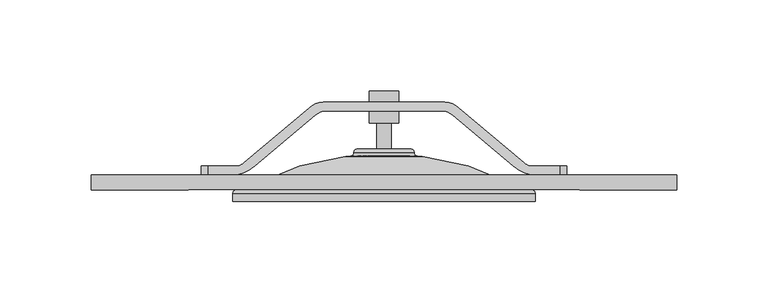
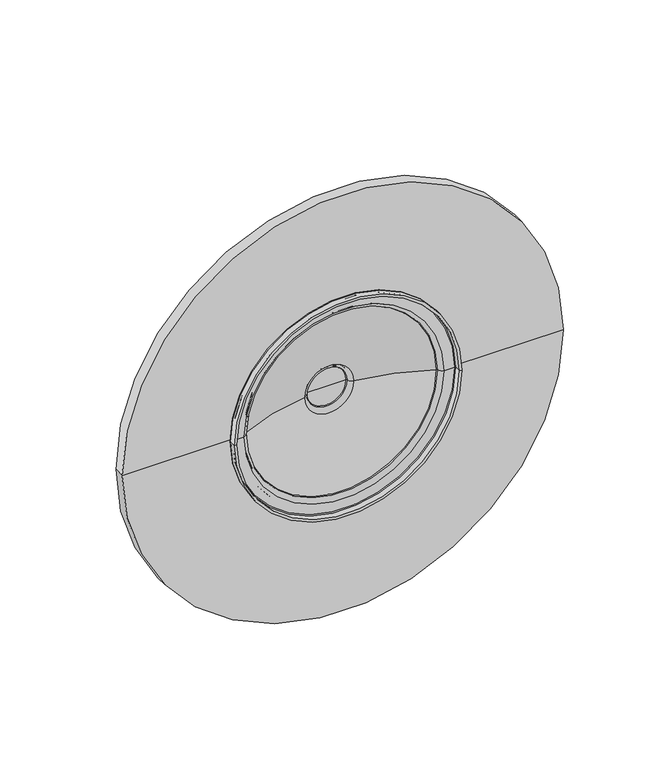
"""IFC4 building model written with IfcOpenShell, lengths in millimetres: proxy geometry, BVNC 300 8Y. : BVNC 300 8Y."""

from ifc_helpers import new_model, si_unit, point, frame, origin, place, context, project, spatial, polyline, circle_curve, ellipse_curve, trimmed, source, transform, mapped, element, save
from ifc_brep_helpers import plane_surface, cylinder_surface, revolved_surface, advanced_brep


def mechanical_equipment_0f1aea58(model_context):
    return source(origin(), model_context, "Body", "AdvancedBrep", [
        advanced_brep(
        [(44.3795006, 108.0, 2710.0), (54.2298211, 113.0, 2710.0), (87.44309, 140.8692417, 2710.0), (91.8102497, 143.0, 2710.0), (125.0, 143.0, 2710.0), (158.1897503, 143.0, 2710.0), (162.55691, 140.8692417, 2710.0), (195.7701789, 113.0, 2710.0), (205.6204994, 108.0, 2710.0), (221.2200072, 108.0, 2710.0), (221.2200072, 113.0, 2710.0), (205.6204994, 113.0, 2710.0), (201.5540671, 114.8851429, 2710.0), (165.874925, 144.8234979, 2710.0), (158.1897503, 148.0, 2710.0), (125.0, 148.0, 2710.0), (91.8102497, 148.0, 2710.0), (84.125075, 144.8234979, 2710.0), (48.4459329, 114.8851429, 2710.0), (44.3795006, 113.0, 2710.0), (28.7799928, 113.0, 2710.0), (28.7799928, 108.0, 2710.0), (44.3795006, 113.0, 2690.0), (48.4459329, 114.8851429, 2690.0), (84.125075, 144.8234979, 2690.0), (91.8102497, 148.0, 2690.0), (125.0, 148.0, 2690.0), (158.1897503, 148.0, 2690.0), (165.874925, 144.8234979, 2690.0), (201.5540671, 114.8851429, 2690.0), (205.6204994, 113.0, 2690.0), (221.2200072, 113.0, 2690.0), (221.2200072, 108.0, 2690.0), (205.6204994, 108.0, 2690.0), (195.7701789, 113.0, 2690.0), (162.55691, 140.8692417, 2690.0), (158.1897503, 143.0, 2690.0), (125.0, 143.0, 2690.0), (91.8102497, 143.0, 2690.0), (87.44309, 140.8692417, 2690.0), (54.2298211, 113.0, 2690.0), (44.3795006, 108.0, 2690.0), (28.7799928, 108.0, 2690.0), (28.7799928, 113.0, 2690.0), (25.0, 108.0, 2706.2200072), (25.0, 108.0, 2693.7799928), (225.0, 108.0, 2693.7799928), (225.0, 108.0, 2706.2200072), (225.0, 113.0, 2693.7799928), (225.0, 113.0, 2706.2200072), (25.0, 113.0, 2693.7799928), (25.0, 113.0, 2706.2200072)],
        [
            (0, 1, circle_curve(frame((38.5511411, 131.6851233, 2710.0), z_axis=(0.0, 0.0, 1.0), x_axis=(1.0, 0.0, 0.0)), 24.3916961)),
            (1, 2),
            (2, 3, circle_curve(frame((93.9022065, 133.1715663, 2710.0), z_axis=(0.0, 0.0, -1.0), x_axis=(1.0, 0.0, 0.0)), 10.0486015)),
            (3, 4),
            (4, 5),
            (5, 6, circle_curve(frame((156.0977935, 133.1715663, 2710.0), z_axis=(0.0, 0.0, -1.0), x_axis=(-1.0, 0.0, 0.0)), 10.0486015)),
            (6, 7),
            (7, 8, circle_curve(frame((211.4488589, 131.6851233, 2710.0), z_axis=(0.0, 0.0, 1.0), x_axis=(-1.0, 0.0, 0.0)), 24.3916961)),
            (8, 9),
            (9, 10),
            (10, 11),
            (11, 12, circle_curve(frame((205.6204994, 118.3284116, 2710.0), z_axis=(0.0, 0.0, -1.0), x_axis=(-1.0, 0.0, 0.0)), 5.3284116)),
            (12, 13),
            (13, 14, circle_curve(frame((158.1897503, 137.115059, 2710.0), z_axis=(0.0, 0.0, 1.0), x_axis=(-1.0, 0.0, 0.0)), 10.884941)),
            (14, 15),
            (15, 16),
            (16, 17, circle_curve(frame((91.8102497, 137.115059, 2710.0), z_axis=(0.0, 0.0, 1.0), x_axis=(1.0, 0.0, 0.0)), 10.884941)),
            (17, 18),
            (18, 19, circle_curve(frame((44.3795006, 118.3284116, 2710.0), z_axis=(0.0, 0.0, -1.0), x_axis=(1.0, 0.0, 0.0)), 5.3284116)),
            (19, 20),
            (20, 21),
            (21, 0),
            (22, 23, circle_curve(frame((44.3795006, 118.3284116, 2690.0), z_axis=(0.0, 0.0, 1.0), x_axis=(1.0, 0.0, 0.0)), 5.3284116)),
            (23, 24),
            (24, 25, circle_curve(frame((91.8102497, 137.115059, 2690.0), z_axis=(0.0, 0.0, -1.0), x_axis=(1.0, 0.0, 0.0)), 10.884941)),
            (25, 26),
            (26, 27),
            (27, 28, circle_curve(frame((158.1897503, 137.115059, 2690.0), z_axis=(0.0, 0.0, -1.0), x_axis=(-1.0, 0.0, 0.0)), 10.884941)),
            (28, 29),
            (29, 30, circle_curve(frame((205.6204994, 118.3284116, 2690.0), z_axis=(0.0, 0.0, 1.0), x_axis=(-1.0, 0.0, 0.0)), 5.3284116)),
            (30, 31),
            (31, 32),
            (32, 33),
            (33, 34, circle_curve(frame((211.4488589, 131.6851233, 2690.0), z_axis=(0.0, 0.0, -1.0), x_axis=(-1.0, 0.0, 0.0)), 24.3916961)),
            (34, 35),
            (35, 36, circle_curve(frame((156.0977935, 133.1715663, 2690.0), z_axis=(0.0, 0.0, 1.0), x_axis=(-1.0, 0.0, 0.0)), 10.0486015)),
            (36, 37),
            (37, 38),
            (38, 39, circle_curve(frame((93.9022065, 133.1715663, 2690.0), z_axis=(0.0, 0.0, 1.0), x_axis=(1.0, 0.0, 0.0)), 10.0486015)),
            (39, 40),
            (40, 41, circle_curve(frame((38.5511411, 131.6851233, 2690.0), z_axis=(0.0, 0.0, -1.0), x_axis=(1.0, 0.0, 0.0)), 24.3916961)),
            (41, 42),
            (42, 43),
            (43, 22),
            (41, 0),
            (21, 44, circle_curve(frame((28.7799928, 108.0, 2706.2200072), z_axis=(0.0, -1.0, 0.0), x_axis=(1.0, 0.0, 0.0)), 3.7799928)),
            (44, 45),
            (45, 42, circle_curve(frame((28.7799928, 108.0, 2693.7799928), z_axis=(0.0, -1.0, 0.0), x_axis=(1.0, 0.0, 0.0)), 3.7799928)),
            (40, 1),
            (39, 2),
            (38, 3),
            (37, 4),
            (36, 5),
            (35, 6),
            (34, 7),
            (33, 8),
            (32, 46, circle_curve(frame((221.2200072, 108.0, 2693.7799928), z_axis=(0.0, -1.0, 0.0), x_axis=(-1.0, 0.0, 0.0)), 3.7799928)),
            (46, 47),
            (47, 9, circle_curve(frame((221.2200072, 108.0, 2706.2200072), z_axis=(0.0, -1.0, 0.0), x_axis=(-1.0, 0.0, 0.0)), 3.7799928)),
            (46, 48),
            (48, 49),
            (49, 47),
            (30, 11),
            (10, 49, circle_curve(frame((221.2200072, 113.0, 2706.2200072), z_axis=(0.0, 1.0, 0.0), x_axis=(-1.0, 0.0, 0.0)), 3.7799928)),
            (48, 31, circle_curve(frame((221.2200072, 113.0, 2693.7799928), z_axis=(0.0, 1.0, 0.0), x_axis=(-1.0, 0.0, 0.0)), 3.7799928)),
            (29, 12),
            (28, 13),
            (27, 14),
            (26, 15),
            (25, 16),
            (24, 17),
            (23, 18),
            (22, 19),
            (43, 50, circle_curve(frame((28.7799928, 113.0, 2693.7799928), z_axis=(0.0, 1.0, 0.0), x_axis=(1.0, 0.0, 0.0)), 3.7799928)),
            (50, 51),
            (51, 20, circle_curve(frame((28.7799928, 113.0, 2706.2200072), z_axis=(0.0, 1.0, 0.0), x_axis=(1.0, 0.0, 0.0)), 3.7799928)),
            (44, 51),
            (50, 45),
        ],
        [
            plane_surface(frame((25.0, 108.0, 2710.0), z_axis=(0.0, 0.0, 1.0), x_axis=(1.0, 0.0, 0.0))),
            plane_surface(frame((25.0, 108.0, 2690.0), z_axis=(0.0, 0.0, -1.0), x_axis=(-1.0, 0.0, 0.0))),
            plane_surface(frame((25.0, 108.0, 2710.0), z_axis=(0.0, -1.0, 0.0), x_axis=(0.0, 0.0, -1.0))),
            cylinder_surface(frame((38.5511411, 131.6851233, 2690.0), z_axis=(0.0, 0.0, 1.0), x_axis=(1.0, 0.0, 0.0)), 24.3916961),
            plane_surface(frame((54.2298211, 113.0, 2710.0), z_axis=(0.6427876096865391, -0.7660444431189783, 0.0), x_axis=(0.0, 0.0, -1.0))),
            revolved_surface(polyline([(103.95080800000001, 133.1715663, 2690.0), (103.95080800000001, 133.1715663, 2710.0)]), (93.9022065, 133.1715663, 2690.0), (0.0, 0.0, -1.0)),
            plane_surface(frame((91.8102497, 143.0, 2710.0), z_axis=(0.0, -1.0, 0.0), x_axis=(0.0, 0.0, -1.0))),
            plane_surface(frame((125.0, 143.0, 2710.0), z_axis=(0.0, -1.0, 0.0), x_axis=(0.0, 0.0, -1.0))),
            revolved_surface(polyline([(146.049192, 133.1715663, 2690.0), (146.049192, 133.1715663, 2710.0)]), (156.0977935, 133.1715663, 2690.0), (0.0, 0.0, -1.0)),
            plane_surface(frame((162.55691, 140.8692417, 2710.0), z_axis=(-0.6427876096865387, -0.7660444431189786, 0.0), x_axis=(0.0, 0.0, -1.0))),
            cylinder_surface(frame((211.4488589, 131.6851233, 2690.0), z_axis=(0.0, 0.0, 1.0), x_axis=(-1.0, 0.0, 0.0)), 24.3916961),
            plane_surface(frame((205.6204994, 108.0, 2710.0), z_axis=(0.0, -1.0, 0.0), x_axis=(0.0, 0.0, -1.0))),
            plane_surface(frame((225.0, 108.0, 2710.0), z_axis=(1.0, 0.0, 0.0), x_axis=(0.0, 0.0, -1.0))),
            plane_surface(frame((225.0, 113.0, 2710.0), z_axis=(0.0, 1.0, 0.0), x_axis=(0.0, 0.0, -1.0))),
            revolved_surface(polyline([(200.2920878, 118.3284116, 2690.0), (200.2920878, 118.3284116, 2710.0)]), (205.6204994, 118.3284116, 2690.0), (0.0, 0.0, -1.0)),
            plane_surface(frame((201.5540671, 114.8851429, 2710.0), z_axis=(0.6427876096865414, 0.7660444431189763, 0.0), x_axis=(0.0, 0.0, -1.0))),
            cylinder_surface(frame((158.1897503, 137.115059, 2690.0), z_axis=(0.0, 0.0, 1.0), x_axis=(-1.0, 0.0, 0.0)), 10.884941),
            plane_surface(frame((158.1897503, 148.0, 2710.0), z_axis=(0.0, 1.0, 0.0), x_axis=(0.0, 0.0, -1.0))),
            plane_surface(frame((125.0, 148.0, 2710.0), z_axis=(0.0, 1.0, 0.0), x_axis=(0.0, 0.0, -1.0))),
            cylinder_surface(frame((91.8102497, 137.115059, 2690.0), z_axis=(0.0, 0.0, 1.0), x_axis=(1.0, 0.0, 0.0)), 10.884941),
            plane_surface(frame((84.125075, 144.8234979, 2710.0), z_axis=(-0.6427876096865359, 0.766044443118981, 0.0), x_axis=(0.0, 0.0, -1.0))),
            revolved_surface(polyline([(49.7079122, 118.3284116, 2690.0), (49.7079122, 118.3284116, 2710.0)]), (44.3795006, 118.3284116, 2690.0), (0.0, 0.0, -1.0)),
            plane_surface(frame((44.3795006, 113.0, 2710.0), z_axis=(0.0, 1.0, 0.0), x_axis=(0.0, 0.0, -1.0))),
            plane_surface(frame((25.0, 113.0, 2710.0), z_axis=(-1.0, 0.0, 0.0), x_axis=(0.0, 0.0, -1.0))),
            cylinder_surface(frame((28.7799928, 108.0, 2693.7799928), z_axis=(0.0, -1.0, 0.0), x_axis=(1.0, 0.0, 0.0)), 3.7799928),
            cylinder_surface(frame((28.7799928, 93.5, 2706.2200072), z_axis=(0.0, -1.0, 0.0), x_axis=(1.0, 0.0, 0.0)), 3.7799928),
            cylinder_surface(frame((221.2200072, 93.5, 2693.7799928), z_axis=(0.0, -1.0, 0.0), x_axis=(-1.0, 0.0, 0.0)), 3.7799928),
            cylinder_surface(frame((221.2200072, 93.5, 2706.2200072), z_axis=(0.0, -1.0, 0.0), x_axis=(-1.0, 0.0, 0.0)), 3.7799928),
        ],
        [
            (0, [[1, 2, 3, 4, 5, 6, 7, 8, 9, 10, 11, 12, 13, 14, 15, 16, 17, 18, 19, 20, 21, 22]]),
            (1, [[23, 24, 25, 26, 27, 28, 29, 30, 31, 32, 33, 34, 35, 36, 37, 38, 39, 40, 41, 42, 43, 44]]),
            (2, [[45, -22, 46, 47, 48, -42]]),
            (3, [[-1, -45, -41, 49]]),
            (4, [[-2, -49, -40, 50]]),
            (5, [[-3, -50, -39, 51]]),
            (6, [[-4, -51, -38, 52]]),
            (7, [[-5, -52, -37, 53]]),
            (8, [[-6, -53, -36, 54]]),
            (9, [[-7, -54, -35, 55]]),
            (10, [[-8, -55, -34, 56]]),
            (11, [[-56, -33, 57, 58, 59, -9]]),
            (12, [[-58, 60, 61, 62]]),
            (13, [[63, -11, 64, -61, 65, -31]]),
            (14, [[-12, -63, -30, 66]]),
            (15, [[-13, -66, -29, 67]]),
            (16, [[-14, -67, -28, 68]]),
            (17, [[-15, -68, -27, 69]]),
            (18, [[-16, -69, -26, 70]]),
            (19, [[-17, -70, -25, 71]]),
            (20, [[-18, -71, -24, 72]]),
            (21, [[-19, -72, -23, 73]]),
            (22, [[-73, -44, 74, 75, 76, -20]]),
            (23, [[-47, 77, -75, 78]]),
            (24, [[-43, -48, -78, -74]]),
            (25, [[-21, -76, -77, -46]]),
            (26, [[-32, -65, -60, -57]]),
            (27, [[-10, -59, -62, -64]]),
        ],
    ),
        advanced_brep(
        [(207.7271571, 93.5, 2700.0), (42.2728429, 93.5, 2700.0), (42.2728429, 97.7728429, 2700.0), (207.7271571, 97.7728429, 2700.0), (205.9367462, 93.5, 2700.0), (44.0632538, 93.5, 2700.0), (205.9367462, 97.9071057, 2700.0), (44.0632538, 97.9071057, 2700.0), (205.3438519, 98.5, 2700.0), (44.6561481, 98.5, 2700.0), (197.7785514, 98.5, 2700.0), (52.2214486, 98.5, 2700.0), (194.5390342, 101.1233093, 2700.0), (55.4609658, 101.1233093, 2700.0), (194.110594, 101.9290881, 2700.0), (55.889406, 101.9290881, 2700.0), (143.1174907, 117.056758, 2700.0), (106.8825093, 117.056758, 2700.0), (139.9690463, 120.2052024, 2700.0), (110.0309537, 120.2052024, 2700.0), (139.3942487, 120.78, 2700.0), (110.6057513, 120.78, 2700.0), (125.0, 120.78, 2700.0), (139.6388233, 122.2731901, 2700.0), (110.3611767, 122.2731901, 2700.0), (120.9566338, 122.2731901, 2700.0), (129.0433662, 122.2731901, 2700.0), (141.5029828, 120.4090307, 2700.0), (108.4970172, 120.4090307, 2700.0), (143.1991524, 118.522856, 2700.0), (106.8008476, 118.522856, 2700.0), (145.9642188, 118.2410596, 2700.0), (104.0357812, 118.2410596, 2700.0), (194.877574, 103.206216, 2700.0), (55.122426, 103.206216, 2700.0), (196.1038029, 101.6367146, 2700.0), (53.8961971, 101.6367146, 2700.0), (198.0543634, 100.0, 2700.0), (51.9456366, 100.0, 2700.0), (200.0, 100.0, 2700.0), (50.0, 100.0, 2700.0), (200.0, 108.0, 2700.0), (50.0, 108.0, 2700.0), (285.0, 108.0, 2700.0), (-35.0, 108.0, 2700.0), (285.0, 100.0, 2700.0), (-35.0, 100.0, 2700.0), (205.5, 100.0, 2700.0), (44.5, 100.0, 2700.0), (133.0867323, 136.6576943, 2700.0), (116.9132677, 136.6576943, 2700.0), (116.9132677, 153.9, 2700.0), (133.0867323, 153.9, 2700.0), (129.0433662, 136.6576943, 2700.0), (120.9566338, 136.6576943, 2700.0), (125.0, 153.9, 2700.0)],
        [
            (0, 1, circle_curve(frame((125.0, 93.5, 2700.0), z_axis=(0.0, 1.0, 0.0), x_axis=(-1.0, 0.0, 0.0)), 82.7271571)),
            (1, 2),
            (2, 3, circle_curve(frame((125.0, 97.7728429, 2700.0), z_axis=(0.0, -1.0, 0.0), x_axis=(-1.0, 0.0, 0.0)), 82.7271571)),
            (3, 0),
            (1, 0, circle_curve(frame((125.0, 93.5, 2700.0), z_axis=(0.0, 1.0, 0.0), x_axis=(-1.0, 0.0, 0.0)), 82.7271571)),
            (3, 2, circle_curve(frame((125.0, 97.7728429, 2700.0), z_axis=(0.0, -1.0, 0.0), x_axis=(-1.0, 0.0, 0.0)), 82.7271571)),
            (0, 4),
            (4, 5, circle_curve(frame((125.0, 93.5, 2700.0), z_axis=(0.0, 1.0, 0.0), x_axis=(-1.0, 0.0, 0.0)), 80.9367462)),
            (5, 1),
            (5, 4, circle_curve(frame((125.0, 93.5, 2700.0), z_axis=(0.0, 1.0, 0.0), x_axis=(-1.0, 0.0, 0.0)), 80.9367462)),
            (4, 6),
            (6, 7, circle_curve(frame((125.0, 97.9071057, 2700.0), z_axis=(0.0, 1.0, 0.0), x_axis=(-1.0, 0.0, 0.0)), 80.9367462)),
            (7, 5),
            (7, 6, circle_curve(frame((125.0, 97.9071057, 2700.0), z_axis=(0.0, 1.0, 0.0), x_axis=(-1.0, 0.0, 0.0)), 80.9367462)),
            (6, 8, circle_curve(frame((205.3438519, 97.9071057, 2700.0), z_axis=(0.0, 0.0, 1.0), x_axis=(-1.0, 0.0, 0.0)), 0.5928943)),
            (8, 9, circle_curve(frame((125.0, 98.5, 2700.0), z_axis=(0.0, 1.0, 0.0), x_axis=(-1.0, 0.0, 0.0)), 80.3438519)),
            (9, 7, circle_curve(frame((44.6561481, 97.9071057, 2700.0), z_axis=(0.0, 0.0, 1.0), x_axis=(1.0, 0.0, 0.0)), 0.5928943)),
            (9, 8, circle_curve(frame((125.0, 98.5, 2700.0), z_axis=(0.0, 1.0, 0.0), x_axis=(-1.0, 0.0, 0.0)), 80.3438519)),
            (8, 10),
            (10, 11, circle_curve(frame((125.0, 98.5, 2700.0), z_axis=(0.0, 1.0, 0.0), x_axis=(-1.0, 0.0, 0.0)), 72.7785514)),
            (11, 9),
            (11, 10, circle_curve(frame((125.0, 98.5, 2700.0), z_axis=(0.0, 1.0, 0.0), x_axis=(-1.0, 0.0, 0.0)), 72.7785514)),
            (10, 12, circle_curve(frame((197.9467336, 102.0195777, 2700.0), z_axis=(0.0, 0.0, -1.0), x_axis=(-1.0, 0.0, 0.0)), 3.5235937)),
            (12, 13, circle_curve(frame((125.0, 101.1233093, 2700.0), z_axis=(0.0, 1.0, 0.0), x_axis=(-1.0, 0.0, 0.0)), 69.5390342)),
            (13, 11, circle_curve(frame((52.0532664, 102.0195777, 2700.0), z_axis=(0.0, 0.0, -1.0), x_axis=(1.0, 0.0, 0.0)), 3.5235937)),
            (13, 12, circle_curve(frame((125.0, 101.1233093, 2700.0), z_axis=(0.0, 1.0, 0.0), x_axis=(-1.0, 0.0, 0.0)), 69.5390342)),
            (12, 14, circle_curve(frame((193.7458269, 101.2183458, 2700.0), z_axis=(0.0, 0.0, 1.0), x_axis=(-1.0, 0.0, 0.0)), 0.7988803)),
            (14, 15, circle_curve(frame((125.0, 101.9290881, 2700.0), z_axis=(0.0, 1.0, 0.0), x_axis=(-1.0, 0.0, 0.0)), 69.110594)),
            (15, 13, circle_curve(frame((56.2541731, 101.2183458, 2700.0), z_axis=(0.0, 0.0, 1.0), x_axis=(1.0, 0.0, 0.0)), 0.7988803)),
            (15, 14, circle_curve(frame((125.0, 101.9290881, 2700.0), z_axis=(0.0, 1.0, 0.0), x_axis=(-1.0, 0.0, 0.0)), 69.110594)),
            (14, 16, circle_curve(frame((128.3688639, -26.1675298, 2700.0), z_axis=(0.0, 0.0, 1.0), x_axis=(-1.0, 0.0, 0.0)), 143.9816606)),
            (16, 17, circle_curve(frame((125.0, 117.056758, 2700.0), z_axis=(0.0, 1.0, 0.0), x_axis=(-1.0, 0.0, 0.0)), 18.1174907)),
            (17, 15, circle_curve(frame((121.6311361, -26.1675298, 2700.0), z_axis=(0.0, 0.0, 1.0), x_axis=(1.0, 0.0, 0.0)), 143.9816606)),
            (17, 16, circle_curve(frame((125.0, 117.056758, 2700.0), z_axis=(0.0, 1.0, 0.0), x_axis=(-1.0, 0.0, 0.0)), 18.1174907)),
            (16, 18, circle_curve(frame((143.1174907, 120.2052024, 2700.0), z_axis=(0.0, 0.0, -1.0), x_axis=(-1.0, 0.0, 0.0)), 3.1484444)),
            (18, 19, circle_curve(frame((125.0, 120.2052024, 2700.0), z_axis=(0.0, 1.0, 0.0), x_axis=(-1.0, 0.0, 0.0)), 14.9690463)),
            (19, 17, circle_curve(frame((106.8825093, 120.2052024, 2700.0), z_axis=(0.0, 0.0, -1.0), x_axis=(1.0, 0.0, 0.0)), 3.1484444)),
            (19, 18, circle_curve(frame((125.0, 120.2052024, 2700.0), z_axis=(0.0, 1.0, 0.0), x_axis=(-1.0, 0.0, 0.0)), 14.9690463)),
            (18, 20, circle_curve(frame((139.3942487, 120.2052024, 2700.0), z_axis=(0.0, 0.0, 1.0), x_axis=(-1.0, 0.0, 0.0)), 0.5747976)),
            (20, 21, circle_curve(frame((125.0, 120.78, 2700.0), z_axis=(0.0, 1.0, 0.0), x_axis=(-1.0, 0.0, 0.0)), 14.3942487)),
            (21, 19, circle_curve(frame((110.6057513, 120.2052024, 2700.0), z_axis=(0.0, 0.0, 1.0), x_axis=(1.0, 0.0, 0.0)), 0.5747976)),
            (21, 20, circle_curve(frame((125.0, 120.78, 2700.0), z_axis=(0.0, 1.0, 0.0), x_axis=(-1.0, 0.0, 0.0)), 14.3942487)),
            (20, 22),
            (22, 21),
            (23, 24, circle_curve(frame((125.0, 122.2731901, 2700.0), z_axis=(0.0, 1.0, 0.0), x_axis=(-1.0, 0.0, 0.0)), 14.6388233)),
            (24, 25),
            (25, 26, circle_curve(frame((125.0, 122.2731901, 2700.0), z_axis=(0.0, -1.0, 0.0), x_axis=(-1.0, 0.0, 0.0)), 4.0433662)),
            (26, 23),
            (24, 23, circle_curve(frame((125.0, 122.2731901, 2700.0), z_axis=(0.0, 1.0, 0.0), x_axis=(-1.0, 0.0, 0.0)), 14.6388233)),
            (26, 25, circle_curve(frame((125.0, 122.2731901, 2700.0), z_axis=(0.0, -1.0, 0.0), x_axis=(-1.0, 0.0, 0.0)), 4.0433662)),
            (23, 27, circle_curve(frame((139.6388233, 120.4090307, 2700.0), z_axis=(0.0, 0.0, -1.0), x_axis=(-1.0, 0.0, 0.0)), 1.8641595)),
            (27, 28, circle_curve(frame((125.0, 120.4090307, 2700.0), z_axis=(0.0, 1.0, 0.0), x_axis=(-1.0, 0.0, 0.0)), 16.5029828)),
            (28, 24, circle_curve(frame((110.3611767, 120.4090307, 2700.0), z_axis=(0.0, 0.0, -1.0), x_axis=(1.0, 0.0, 0.0)), 1.8641595)),
            (28, 27, circle_curve(frame((125.0, 120.4090307, 2700.0), z_axis=(0.0, 1.0, 0.0), x_axis=(-1.0, 0.0, 0.0)), 16.5029828)),
            (27, 29, circle_curve(frame((143.3997997, 120.4090307, 2700.0), z_axis=(0.0, 0.0, 1.0), x_axis=(-1.0, 0.0, 0.0)), 1.8968169)),
            (29, 30, circle_curve(frame((125.0, 118.522856, 2700.0), z_axis=(0.0, 1.0, 0.0), x_axis=(-1.0, 0.0, 0.0)), 18.1991524)),
            (30, 28, circle_curve(frame((106.6002003, 120.4090307, 2700.0), z_axis=(0.0, 0.0, 1.0), x_axis=(1.0, 0.0, 0.0)), 1.8968169)),
            (30, 29, circle_curve(frame((125.0, 118.522856, 2700.0), z_axis=(0.0, 1.0, 0.0), x_axis=(-1.0, 0.0, 0.0)), 18.1991524)),
            (29, 31, circle_curve(frame((176.4809645, 431.386753, 2700.0), z_axis=(0.0, 0.0, 1.0), x_axis=(-1.0, 0.0, 0.0)), 314.6291421)),
            (31, 32, circle_curve(frame((125.0, 118.2410596, 2700.0), z_axis=(0.0, 1.0, 0.0), x_axis=(-1.0, 0.0, 0.0)), 20.9642188)),
            (32, 30, circle_curve(frame((73.5190355, 431.386753, 2700.0), z_axis=(0.0, 0.0, 1.0), x_axis=(1.0, 0.0, 0.0)), 314.6291421)),
            (32, 31, circle_curve(frame((125.0, 118.2410596, 2700.0), z_axis=(0.0, 1.0, 0.0), x_axis=(-1.0, 0.0, 0.0)), 20.9642188)),
            (31, 33, circle_curve(frame((131.9555378, -14.4169888, 2700.0), z_axis=(0.0, 0.0, -1.0), x_axis=(-1.0, 0.0, 0.0)), 133.3956557)),
            (33, 34, circle_curve(frame((125.0, 103.206216, 2700.0), z_axis=(0.0, 1.0, 0.0), x_axis=(-1.0, 0.0, 0.0)), 69.877574)),
            (34, 32, circle_curve(frame((118.0444622, -14.4169888, 2700.0), z_axis=(0.0, 0.0, -1.0), x_axis=(1.0, 0.0, 0.0)), 133.3956557)),
            (34, 33, circle_curve(frame((125.0, 103.206216, 2700.0), z_axis=(0.0, 1.0, 0.0), x_axis=(-1.0, 0.0, 0.0)), 69.877574)),
            (33, 35, circle_curve(frame((194.0147871, 101.2683648, 2700.0), z_axis=(0.0, 0.0, -1.0), x_axis=(-1.0, 0.0, 0.0)), 2.1212422)),
            (35, 36, circle_curve(frame((125.0, 101.6367146, 2700.0), z_axis=(0.0, 1.0, 0.0), x_axis=(-1.0, 0.0, 0.0)), 71.1038029)),
            (36, 34, circle_curve(frame((55.9852129, 101.2683648, 2700.0), z_axis=(0.0, 0.0, -1.0), x_axis=(1.0, 0.0, 0.0)), 2.1212422)),
            (36, 35, circle_curve(frame((125.0, 101.6367146, 2700.0), z_axis=(0.0, 1.0, 0.0), x_axis=(-1.0, 0.0, 0.0)), 71.1038029)),
            (35, 37, circle_curve(frame((198.0543634, 101.9806511, 2700.0), z_axis=(0.0, 0.0, 1.0), x_axis=(-1.0, 0.0, 0.0)), 1.9806511)),
            (37, 38, circle_curve(frame((125.0, 100.0, 2700.0), z_axis=(0.0, 1.0, 0.0), x_axis=(-1.0, 0.0, 0.0)), 73.0543634)),
            (38, 36, circle_curve(frame((51.9456366, 101.9806511, 2700.0), z_axis=(0.0, 0.0, 1.0), x_axis=(1.0, 0.0, 0.0)), 1.9806511)),
            (38, 37, circle_curve(frame((125.0, 100.0, 2700.0), z_axis=(0.0, 1.0, 0.0), x_axis=(-1.0, 0.0, 0.0)), 73.0543634)),
            (37, 39),
            (39, 40, circle_curve(frame((125.0, 100.0, 2700.0), z_axis=(0.0, 1.0, 0.0), x_axis=(-1.0, 0.0, 0.0)), 75.0)),
            (40, 38),
            (40, 39, circle_curve(frame((125.0, 100.0, 2700.0), z_axis=(0.0, 1.0, 0.0), x_axis=(-1.0, 0.0, 0.0)), 75.0)),
            (39, 41),
            (41, 42, circle_curve(frame((125.0, 108.0, 2700.0), z_axis=(0.0, 1.0, 0.0), x_axis=(-1.0, 0.0, 0.0)), 75.0)),
            (42, 40),
            (42, 41, circle_curve(frame((125.0, 108.0, 2700.0), z_axis=(0.0, 1.0, 0.0), x_axis=(-1.0, 0.0, 0.0)), 75.0)),
            (41, 43),
            (43, 44, circle_curve(frame((125.0, 108.0, 2700.0), z_axis=(0.0, 1.0, 0.0), x_axis=(-1.0, 0.0, 0.0)), 160.0)),
            (44, 42),
            (44, 43, circle_curve(frame((125.0, 108.0, 2700.0), z_axis=(0.0, 1.0, 0.0), x_axis=(-1.0, 0.0, 0.0)), 160.0)),
            (43, 45),
            (45, 46, circle_curve(frame((125.0, 100.0, 2700.0), z_axis=(0.0, 1.0, 0.0), x_axis=(-1.0, 0.0, 0.0)), 160.0)),
            (46, 44),
            (46, 45, circle_curve(frame((125.0, 100.0, 2700.0), z_axis=(0.0, 1.0, 0.0), x_axis=(-1.0, 0.0, 0.0)), 160.0)),
            (45, 47),
            (47, 48, circle_curve(frame((125.0, 100.0, 2700.0), z_axis=(0.0, 1.0, 0.0), x_axis=(-1.0, 0.0, 0.0)), 80.5)),
            (48, 46),
            (48, 47, circle_curve(frame((125.0, 100.0, 2700.0), z_axis=(0.0, 1.0, 0.0), x_axis=(-1.0, 0.0, 0.0)), 80.5)),
            (2, 48, circle_curve(frame((44.5, 97.7728429, 2700.0), z_axis=(0.0, 0.0, -1.0), x_axis=(1.0, 0.0, 0.0)), 2.2271571)),
            (47, 3, circle_curve(frame((205.5, 97.7728429, 2700.0), z_axis=(0.0, 0.0, -1.0), x_axis=(-1.0, 0.0, 0.0)), 2.2271571)),
            (49, 50, circle_curve(frame((125.0, 136.6576943, 2700.0), z_axis=(0.0, 1.0, 0.0), x_axis=(-1.0, 0.0, 0.0)), 8.0867323)),
            (50, 51),
            (51, 52, circle_curve(frame((125.0, 153.9, 2700.0), z_axis=(0.0, -1.0, 0.0), x_axis=(-1.0, 0.0, 0.0)), 8.0867323)),
            (52, 49),
            (50, 49, circle_curve(frame((125.0, 136.6576943, 2700.0), z_axis=(0.0, 1.0, 0.0), x_axis=(-1.0, 0.0, 0.0)), 8.0867323)),
            (52, 51, circle_curve(frame((125.0, 153.9, 2700.0), z_axis=(0.0, -1.0, 0.0), x_axis=(-1.0, 0.0, 0.0)), 8.0867323)),
            (49, 53),
            (53, 54, circle_curve(frame((125.0, 136.6576943, 2700.0), z_axis=(0.0, 1.0, 0.0), x_axis=(-1.0, 0.0, 0.0)), 4.0433662)),
            (54, 50),
            (54, 53, circle_curve(frame((125.0, 136.6576943, 2700.0), z_axis=(0.0, 1.0, 0.0), x_axis=(-1.0, 0.0, 0.0)), 4.0433662)),
            (51, 55),
            (55, 52),
            (25, 54),
            (53, 26),
        ],
        [
            cylinder_surface(frame((125.0, 193.5, 2700.0), z_axis=(0.0, -1.0, 0.0), x_axis=(-1.0, 0.0, 0.0)), 82.7271571),
            plane_surface(frame((125.0, 93.5, 2700.0), z_axis=(0.0, -1.0, 0.0), x_axis=(-1.0, 0.0, 0.0))),
            revolved_surface(polyline([(44.0632538, 93.5, 2700.0), (44.0632538, 97.9071057, 2700.0)]), (125.0, 193.5, 2700.0), (0.0, -1.0, 0.0)),
            revolved_surface(trimmed(ellipse_curve(frame((44.6561481, 97.9071057, 2700.0), z_axis=(0.0, 0.0, -1.0), x_axis=(1.0, 0.0, 0.0)), 0.5928943, 0.5928943), [point((44.0632538, 97.9071057, 2700.0))], [point((44.6561481, 98.5, 2700.0))], True, "CARTESIAN"), (125.0, 193.5, 2700.0), (0.0, -1.0, 0.0)),
            plane_surface(frame((125.0, 98.5, 2700.0), z_axis=(0.0, -1.0, 0.0), x_axis=(-1.0, 0.0, 0.0))),
            revolved_surface(trimmed(ellipse_curve(frame((52.0532664, 102.0195777, 2700.0), z_axis=(0.0, 0.0, 1.0), x_axis=(1.0, 0.0, 0.0)), 3.5235937, 3.5235937), [point((52.2214486, 98.5, 2700.0))], [point((55.4609658, 101.1233093, 2700.0))], True, "CARTESIAN"), (125.0, 193.5, 2700.0), (0.0, -1.0, 0.0)),
            revolved_surface(trimmed(ellipse_curve(frame((56.2541731, 101.2183458, 2700.0), z_axis=(0.0, 0.0, -1.0), x_axis=(1.0, 0.0, 0.0)), 0.7988803, 0.7988803), [point((55.4609658, 101.1233093, 2700.0))], [point((55.889406, 101.9290881, 2700.0))], True, "CARTESIAN"), (125.0, 193.5, 2700.0), (0.0, -1.0, 0.0)),
            revolved_surface(trimmed(ellipse_curve(frame((121.6311361, -26.1675298, 2700.0), z_axis=(0.0, 0.0, -1.0), x_axis=(1.0, 0.0, 0.0)), 143.9816606, 143.9816606), [point((55.889406, 101.9290881, 2700.0))], [point((106.8825093, 117.056758, 2700.0))], True, "CARTESIAN"), (125.0, 193.5, 2700.0), (0.0, -1.0, 0.0)),
            revolved_surface(trimmed(ellipse_curve(frame((106.8825093, 120.2052024, 2700.0), z_axis=(0.0, 0.0, 1.0), x_axis=(1.0, 0.0, 0.0)), 3.1484444, 3.1484444), [point((106.8825093, 117.056758, 2700.0))], [point((110.0309537, 120.2052024, 2700.0))], True, "CARTESIAN"), (125.0, 193.5, 2700.0), (0.0, -1.0, 0.0)),
            revolved_surface(trimmed(ellipse_curve(frame((110.6057513, 120.2052024, 2700.0), z_axis=(0.0, 0.0, -1.0), x_axis=(1.0, 0.0, 0.0)), 0.5747976, 0.5747976), [point((110.0309537, 120.2052024, 2700.0))], [point((110.6057513, 120.78, 2700.0))], True, "CARTESIAN"), (125.0, 193.5, 2700.0), (0.0, -1.0, 0.0)),
            plane_surface(frame((125.0, 120.78, 2700.0), z_axis=(0.0, -1.0, 0.0), x_axis=(-1.0, 0.0, 0.0))),
            plane_surface(frame((125.0, 122.2731901, 2700.0), z_axis=(0.0, 1.0, 0.0), x_axis=(-1.0, 0.0, 0.0))),
            revolved_surface(trimmed(ellipse_curve(frame((110.3611767, 120.4090307, 2700.0), z_axis=(0.0, 0.0, 1.0), x_axis=(1.0, 0.0, 0.0)), 1.8641595, 1.8641595), [point((110.3611767, 122.2731901, 2700.0))], [point((108.4970172, 120.4090307, 2700.0))], True, "CARTESIAN"), (125.0, 193.5, 2700.0), (0.0, -1.0, 0.0)),
            revolved_surface(trimmed(ellipse_curve(frame((106.6002003, 120.4090307, 2700.0), z_axis=(0.0, 0.0, -1.0), x_axis=(1.0, 0.0, 0.0)), 1.8968169, 1.8968169), [point((108.4970172, 120.4090307, 2700.0))], [point((106.8008476, 118.522856, 2700.0))], True, "CARTESIAN"), (125.0, 193.5, 2700.0), (0.0, -1.0, 0.0)),
            revolved_surface(trimmed(ellipse_curve(frame((73.5190355, 431.386753, 2700.0), z_axis=(0.0, 0.0, -1.0), x_axis=(1.0, 0.0, 0.0)), 314.6291421, 314.6291421), [point((106.8008476, 118.522856, 2700.0))], [point((104.0357812, 118.2410596, 2700.0))], True, "CARTESIAN"), (125.0, 193.5, 2700.0), (0.0, -1.0, 0.0)),
            revolved_surface(trimmed(ellipse_curve(frame((118.0444622, -14.4169888, 2700.0), z_axis=(0.0, 0.0, 1.0), x_axis=(1.0, 0.0, 0.0)), 133.3956557, 133.3956557), [point((104.0357812, 118.2410596, 2700.0))], [point((55.122426, 103.206216, 2700.0))], True, "CARTESIAN"), (125.0, 193.5, 2700.0), (0.0, -1.0, 0.0)),
            revolved_surface(trimmed(ellipse_curve(frame((55.9852129, 101.2683648, 2700.0), z_axis=(0.0, 0.0, 1.0), x_axis=(1.0, 0.0, 0.0)), 2.1212422, 2.1212422), [point((55.122426, 103.206216, 2700.0))], [point((53.8961971, 101.6367146, 2700.0))], True, "CARTESIAN"), (125.0, 193.5, 2700.0), (0.0, -1.0, 0.0)),
            revolved_surface(trimmed(ellipse_curve(frame((51.9456366, 101.9806511, 2700.0), z_axis=(0.0, 0.0, -1.0), x_axis=(1.0, 0.0, 0.0)), 1.9806511, 1.9806511), [point((53.8961971, 101.6367146, 2700.0))], [point((51.9456366, 100.0, 2700.0))], True, "CARTESIAN"), (125.0, 193.5, 2700.0), (0.0, -1.0, 0.0)),
            plane_surface(frame((125.0, 100.0, 2700.0), z_axis=(0.0, 1.0, 0.0), x_axis=(-1.0, 0.0, 0.0))),
            revolved_surface(polyline([(50.0, 100.0, 2700.0), (50.0, 108.0, 2700.0)]), (125.0, 193.5, 2700.0), (0.0, -1.0, 0.0)),
            plane_surface(frame((125.0, 108.0, 2700.0), z_axis=(0.0, 1.0, 0.0), x_axis=(-1.0, 0.0, 0.0))),
            cylinder_surface(frame((125.0, 193.5, 2700.0), z_axis=(0.0, -1.0, 0.0), x_axis=(-1.0, 0.0, 0.0)), 160.0),
            plane_surface(frame((125.0, 100.0, 2700.0), z_axis=(0.0, -1.0, 0.0), x_axis=(-1.0, 0.0, 0.0))),
            revolved_surface(trimmed(ellipse_curve(frame((44.5, 97.7728429, 2700.0), z_axis=(0.0, 0.0, 1.0), x_axis=(1.0, 0.0, 0.0)), 2.2271571, 2.2271571), [point((44.5, 100.0, 2700.0))], [point((42.2728429, 97.7728429, 2700.0))], True, "CARTESIAN"), (125.0, 193.5, 2700.0), (0.0, -1.0, 0.0)),
            cylinder_surface(frame((125.0, 193.5, 2700.0), z_axis=(0.0, -1.0, 0.0), x_axis=(-1.0, 0.0, 0.0)), 8.0867323),
            plane_surface(frame((125.0, 136.6576943, 2700.0), z_axis=(0.0, -1.0, 0.0), x_axis=(-1.0, 0.0, 0.0))),
            plane_surface(frame((125.0, 153.9, 2700.0), z_axis=(0.0, 1.0, 0.0), x_axis=(-1.0, 0.0, 0.0))),
            cylinder_surface(frame((125.0, 193.5, 2700.0), z_axis=(0.0, -1.0, 0.0), x_axis=(-1.0, 0.0, 0.0)), 4.0433662),
        ],
        [
            (0, [[1, 2, 3, 4]]),
            (0, [[-2, 5, -4, 6]]),
            (1, [[-1, 7, 8, 9]]),
            (1, [[-5, -9, 10, -7]]),
            (2, [[-8, 11, 12, 13]]),
            (2, [[-10, -13, 14, -11]]),
            (3, [[-12, 15, 16, 17]]),
            (3, [[-14, -17, 18, -15]]),
            (4, [[-16, 19, 20, 21]]),
            (4, [[-18, -21, 22, -19]]),
            (5, [[-20, 23, 24, 25]]),
            (5, [[-22, -25, 26, -23]]),
            (6, [[-24, 27, 28, 29]]),
            (6, [[-26, -29, 30, -27]]),
            (7, [[-28, 31, 32, 33]]),
            (7, [[-30, -33, 34, -31]]),
            (8, [[-32, 35, 36, 37]]),
            (8, [[-34, -37, 38, -35]]),
            (9, [[-36, 39, 40, 41]]),
            (9, [[-38, -41, 42, -39]]),
            (10, [[-40, 43, 44]]),
            (10, [[-42, -44, -43]]),
            (11, [[45, 46, 47, 48]]),
            (11, [[-46, 49, -48, 50]]),
            (12, [[-45, 51, 52, 53]]),
            (12, [[-49, -53, 54, -51]]),
            (13, [[-52, 55, 56, 57]]),
            (13, [[-54, -57, 58, -55]]),
            (14, [[-56, 59, 60, 61]]),
            (14, [[-58, -61, 62, -59]]),
            (15, [[-60, 63, 64, 65]]),
            (15, [[-62, -65, 66, -63]]),
            (16, [[-64, 67, 68, 69]]),
            (16, [[-66, -69, 70, -67]]),
            (17, [[-68, 71, 72, 73]]),
            (17, [[-70, -73, 74, -71]]),
            (18, [[-72, 75, 76, 77]]),
            (18, [[-74, -77, 78, -75]]),
            (19, [[-76, 79, 80, 81]]),
            (19, [[-78, -81, 82, -79]]),
            (20, [[-80, 83, 84, 85]]),
            (20, [[-82, -85, 86, -83]]),
            (21, [[-84, 87, 88, 89]]),
            (21, [[-86, -89, 90, -87]]),
            (22, [[-88, 91, 92, 93]]),
            (22, [[-90, -93, 94, -91]]),
            (23, [[-3, 95, -92, 96]]),
            (23, [[-6, -96, -94, -95]]),
            (24, [[97, 98, 99, 100]]),
            (24, [[-98, 101, -100, 102]]),
            (25, [[-97, 103, 104, 105]]),
            (25, [[-101, -105, 106, -103]]),
            (26, [[-99, 107, 108]]),
            (26, [[-102, -108, -107]]),
            (27, [[-47, 109, -104, 110]]),
            (27, [[-50, -110, -106, -109]]),
        ],
    ),
    ])


if __name__ == "__main__":
    model = new_model("IFC4")
    model_context = context("Model", 3, world=origin())
    ifc_project = project(units=[si_unit("LENGTHUNIT", "METRE", prefix="MILLI")], contexts=[model_context])
    site = spatial("IfcSite", under=ifc_project)
    building = spatial("IfcBuilding", under=site)
    placement = place(None, origin())
    mechanical_equipment_shape = mechanical_equipment_0f1aea58(model_context)
    element("IfcBuildingElementProxy", 1, Name="BVNC 300 8Y. : BVNC 300 8Y", ObjectType="BVNC 300 8Y. : BVNC 300 8Y", at=placement, inside=building, context=model_context, shape_type="MappedRepresentation", body=[
        mapped(mechanical_equipment_shape, transform((0.0, 0.0, 0.0), x_axis=(1.0, 0.0, 0.0), y_axis=(0.0, 1.0, 0.0), z_axis=(0.0, 0.0, 1.0))),
    ])
    save(model, "model.ifc")

# Revit data of these elements
# Type "BVNC 300 8Y. : BVNC 300 8Y"
#   Model = "BVNC 300 8Y"
#   FLANGE HEIGHT [instance default] = 2700 mm
#   Default Elevation = 0
